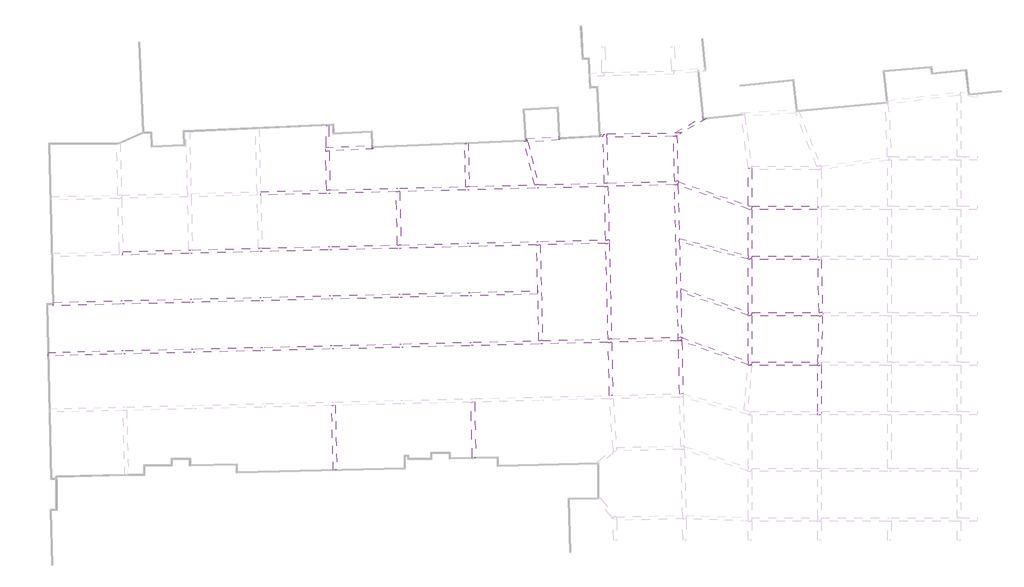
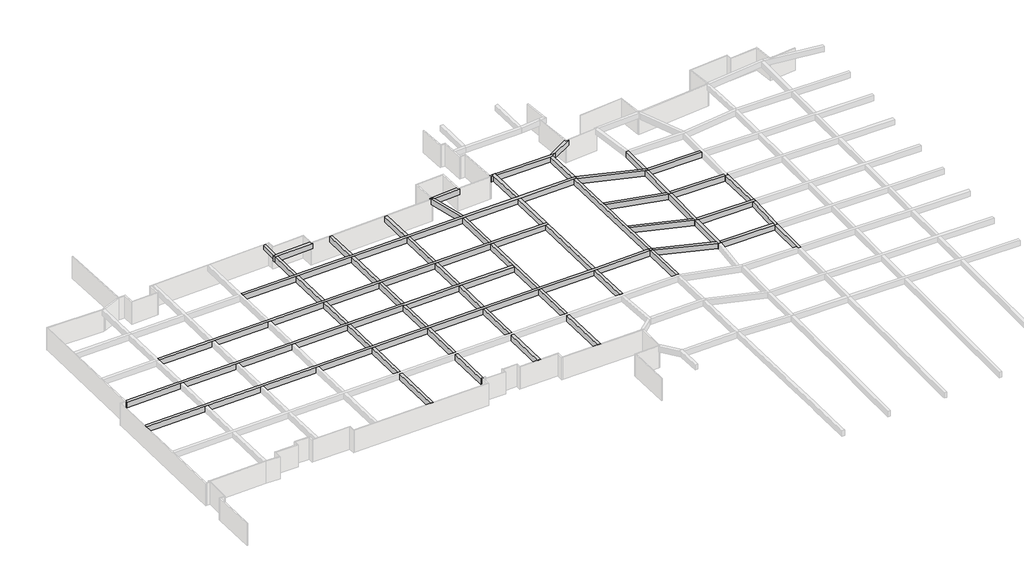
# One storey, part 17 of 20: 39 beams.
"""IFC4 building model written with IfcOpenShell, lengths in millimetres."""

from ifc_helpers import new_model, si_unit, frame, origin, place, context, project, spatial, polyline, outline, extrude, faceted_brep, element, save

model = new_model("IFC4")

# Units and contexts
model_context = context("Model", 3, world=origin())
ifc_project = project(units=[si_unit("LENGTHUNIT", "METRE", prefix="MILLI")], contexts=[model_context])

# Site, building, storey
site = spatial("IfcSite", under=ifc_project)
building = spatial("IfcBuilding", under=site)
storey = spatial("IfcBuildingStorey", under=building, Name="户型图", Elevation=0.0)

# Beams
placement = place(None, origin())
element("IfcBeam", 1, ObjectType="混凝土 - 矩形梁 : KL_beam", at=placement, inside=storey, context=model_context, shape_type="Brep", body=[
    faceted_brep([(46399.9946479, 182003.2647661, 3300.0), (46391.4589732, 182342.894025, 3300.0), (46389.9448891, 182403.1384991, 3300.0), (45990.0711561, 182393.0887404, 3300.0), (38313.3533834, 182200.154934, 3300.0), (37913.4796504, 182190.1051752, 3300.0), (30327.3489539, 181999.4480332, 3300.0), (29917.7537876, 181989.1539522, 3300.0), (22388.2477985, 181799.9199209, 3300.0), (21988.3737022, 181789.8701531, 3300.0), (14385.2020605, 181598.7847323, 3300.0), (13985.327054, 181588.7349416, 3300.0), (6399.8057805, 181398.0931157, 3300.0), (5999.9320475, 181388.043357, 3300.0), (-1606.785957, 181196.8688079, 3300.0), (-1597.0758138, 180796.9865396, 3300.0), (6009.5809432, 180988.1595494, 3300.0), (6409.4554783, 180998.2093283, 3300.0), (13994.367621, 181188.8358453, 3300.0), (14394.2426275, 181198.885636, 3300.0), (21997.9864051, 181389.9854358, 3300.0), (22397.8602787, 181400.0351981, 3300.0), (29976.8508171, 181590.5128914, 3300.0), (30376.7246906, 181600.5626536, 3300.0), (37923.3235545, 181790.2262686, 3300.0), (38323.1974993, 181800.2760327, 3300.0), (45975.016058, 181992.5840638, 3300.0), (46374.889791, 182002.6338225, 3300.0), (46399.9946479, 182003.2647661, 2500.0), (-1597.0758138, 180796.9865396, 2500.0), (6009.5809432, 180988.1595494, 2500.0), (6409.4554783, 180998.2093283, 2500.0), (13994.367621, 181188.8358453, 2500.0), (14394.2426275, 181198.885636, 2500.0), (21997.9864051, 181389.9854358, 2500.0), (22397.8602787, 181400.0351981, 2500.0), (29976.8508171, 181590.5128914, 2500.0), (30376.7246906, 181600.5626536, 2500.0), (37923.3235545, 181790.2262686, 2500.0), (38323.1974993, 181800.2760327, 2500.0), (45975.016058, 181992.5840638, 2500.0), (46374.889791, 182002.6338225, 2500.0), (46389.9448891, 182403.1384991, 2500.0), (46391.4589732, 182342.894025, 2500.0), (-1606.785957, 181196.8688079, 2500.0), (5999.9320475, 181388.043357, 2500.0), (6399.8057805, 181398.0931157, 2500.0), (13985.327054, 181588.7349416, 2500.0), (14385.2020605, 181598.7847323, 2500.0), (21988.3737022, 181789.8701531, 2500.0), (22388.2477985, 181799.9199209, 2500.0), (29917.7537876, 181989.1539522, 2500.0), (30327.3489539, 181999.4480332, 2500.0), (37913.4796504, 182190.1051752, 2500.0), (38313.3533834, 182200.154934, 2500.0), (45990.0711561, 182393.0887404, 2500.0)], [[[0, 1, 2, 3, 4, 5, 6, 7, 8, 9, 10, 11, 12, 13, 14, 15, 16, 17, 18, 19, 20, 21, 22, 23, 24, 25, 26, 27]], [[28, 0, 27, 26, 25, 24, 23, 22, 21, 20, 19, 18, 17, 16, 15, 29, 30, 31, 32, 33, 34, 35, 36, 37, 38, 39, 40, 41]], [[42, 43, 28, 41, 40, 39, 38, 37, 36, 35, 34, 33, 32, 31, 30, 29, 44, 45, 46, 47, 48, 49, 50, 51, 52, 53, 54, 55]], [[2, 42, 55, 54, 53, 52, 51, 50, 49, 48, 47, 46, 45, 44, 14, 13, 12, 11, 10, 9, 8, 7, 6, 5, 4, 3]], [[15, 14, 44, 29]], [[2, 1, 0, 28, 43, 42]]]),
])
element("IfcBeam", 2, ObjectType="混凝土 - 矩形梁 : KL_beam", at=placement, inside=storey, context=model_context, shape_type="Brep", body=[
    faceted_brep([(38480.8232268, 175260.5053635, 3300.0), (38471.1849707, 175660.3892266, 3300.0), (38071.3011075, 175650.7509705, 3300.0), (30525.6842312, 175468.8816956, 3300.0), (30125.8003608, 175459.2434392, 3300.0), (22546.6203468, 175276.5652041, 3300.0), (22146.7364764, 175266.9269478, 3300.0), (14532.4960637, 175083.4036646, 3300.0), (14132.6117538, 175073.7653977, 3300.0), (6550.7038885, 174891.0214142, 3300.0), (6150.8198357, 174881.3831535, 3300.0), (-1448.98219, 174698.2078735, 3300.0), (-1848.8660596, 174688.5696172, 3300.0), (-9443.7780087, 174505.5122009, 3300.0), (-9843.6618727, 174495.8739447, 3300.0), (-17442.3866011, 174312.7246305, 3300.0), (-17432.8215196, 173912.8390036, 3300.0), (-9834.048465, 174095.9894827, 3300.0), (-9434.164601, 174105.6277388, 3300.0), (-1839.1559197, 174288.6874866, 3300.0), (-1439.2720501, 174298.3257429, 3300.0), (6160.0686563, 174481.4899039, 3300.0), (6559.9527091, 174491.1281646, 3300.0), (14141.6523021, 174673.8671282, 3300.0), (14541.5366119, 174683.5053951, 3300.0), (22156.450981, 174867.0449224, 3300.0), (22556.3348514, 174876.6831788, 3300.0), (30135.5148654, 175059.3614139, 3300.0), (30535.3987358, 175068.9996702, 3300.0), (38080.9377827, 175250.8670692, 3300.0), (38480.8232268, 175260.5053635, 2500.0), (-17432.8215196, 173912.8390036, 2500.0), (-9834.048465, 174095.9894827, 2500.0), (-9434.164601, 174105.6277388, 2500.0), (-1839.1559197, 174288.6874866, 2500.0), (-1439.2720501, 174298.3257429, 2500.0), (6160.0686563, 174481.4899039, 2500.0), (6559.9527091, 174491.1281646, 2500.0), (14141.6523021, 174673.8671282, 2500.0), (14541.5366119, 174683.5053951, 2500.0), (22156.450981, 174867.0449224, 2500.0), (22556.3348514, 174876.6831788, 2500.0), (30135.5148654, 175059.3614139, 2500.0), (30535.3987358, 175068.9996702, 2500.0), (38080.9377827, 175250.8670692, 2500.0), (38471.1849707, 175660.3892266, 2500.0), (-17442.3866011, 174312.7246305, 2500.0), (-9843.6618727, 174495.8739447, 2500.0), (-9443.7780087, 174505.5122009, 2500.0), (-1848.8660596, 174688.5696172, 2500.0), (-1448.98219, 174698.2078735, 2500.0), (6150.8198357, 174881.3831535, 2500.0), (6550.7038885, 174891.0214142, 2500.0), (14132.6117538, 175073.7653977, 2500.0), (14532.4960637, 175083.4036646, 2500.0), (22146.7364764, 175266.9269478, 2500.0), (22546.6203468, 175276.5652041, 2500.0), (30125.8003608, 175459.2434392, 2500.0), (30525.6842312, 175468.8816956, 2500.0), (38071.3011075, 175650.7509705, 2500.0)], [[[0, 1, 2, 3, 4, 5, 6, 7, 8, 9, 10, 11, 12, 13, 14, 15, 16, 17, 18, 19, 20, 21, 22, 23, 24, 25, 26, 27, 28, 29]], [[30, 0, 29, 28, 27, 26, 25, 24, 23, 22, 21, 20, 19, 18, 17, 16, 31, 32, 33, 34, 35, 36, 37, 38, 39, 40, 41, 42, 43, 44]], [[45, 30, 44, 43, 42, 41, 40, 39, 38, 37, 36, 35, 34, 33, 32, 31, 46, 47, 48, 49, 50, 51, 52, 53, 54, 55, 56, 57, 58, 59]], [[1, 45, 59, 58, 57, 56, 55, 54, 53, 52, 51, 50, 49, 48, 47, 46, 15, 14, 13, 12, 11, 10, 9, 8, 7, 6, 5, 4, 3, 2]], [[16, 15, 46, 31]], [[1, 0, 30, 45]]]),
])
element("IfcBeam", 3, ObjectType="混凝土 - 矩形梁 : KL_beam", at=placement, inside=storey, context=model_context, shape_type="Brep", body=[
    faceted_brep([(-25454.7766609, 168469.9429507, 3300.0), (-25454.7766609, 168469.9429507, 2500.0), (-25445.2115795, 168070.0573306, 2500.0), (-25445.2115795, 168070.0573306, 3300.0), (-17696.541926, 168255.4019703, 3300.0), (-17296.6562991, 168264.9670519, 3300.0), (-9698.2373562, 168446.7177632, 3300.0), (-9298.3517331, 168456.2828447, 3300.0), (-1701.9427196, 168637.9854794, 3300.0), (-1302.0570732, 168647.5505615, 3300.0), (6290.7968198, 168829.1681594, 3300.0), (6690.682565, 168838.7332438, 3300.0), (14269.4696311, 169020.0143696, 3300.0), (14669.3555953, 169029.5794592, 3300.0), (22293.8325295, 169211.9534658, 3300.0), (22693.7181776, 169221.5185479, 3300.0), (30272.9318843, 169402.8098788, 3300.0), (30263.2173792, 169802.6919248, 3300.0), (22684.0036725, 169621.4005939, 3300.0), (22284.1180244, 169611.8355118, 3300.0), (14660.3150494, 169429.477626, 3300.0), (14260.4290852, 169419.9125364, 3300.0), (6681.4337459, 169238.6264288, 3300.0), (6281.5480006, 169229.0613444, 3300.0), (-1311.7672135, 169047.4327119, 3300.0), (-1711.65286, 169037.8676298, 3300.0), (-9307.9651408, 168856.1673089, 3300.0), (-9707.8507639, 168846.6022274, 3300.0), (-17306.2945554, 168664.8509217, 3300.0), (-17706.1801823, 168655.2858401, 3300.0), (-17696.541926, 168255.4019703, 2500.0), (-17296.6562991, 168264.9670519, 2500.0), (-9698.2373562, 168446.7177632, 2500.0), (-9298.3517331, 168456.2828447, 2500.0), (-1701.9427196, 168637.9854794, 2500.0), (-1302.0570732, 168647.5505615, 2500.0), (6290.7968198, 168829.1681594, 2500.0), (6690.682565, 168838.7332438, 2500.0), (14269.4696311, 169020.0143696, 2500.0), (14669.3555953, 169029.5794592, 2500.0), (22293.8325295, 169211.9534658, 2500.0), (22693.7181776, 169221.5185479, 2500.0), (30272.9318843, 169402.8098788, 2500.0), (-17706.1801823, 168655.2858401, 2500.0), (-17306.2945554, 168664.8509217, 2500.0), (-9707.8507639, 168846.6022274, 2500.0), (-9307.9651408, 168856.1673089, 2500.0), (-1711.65286, 169037.8676298, 2500.0), (-1311.7672135, 169047.4327119, 2500.0), (6281.5480006, 169229.0613444, 2500.0), (6681.4337459, 169238.6264288, 2500.0), (14260.4290852, 169419.9125364, 2500.0), (14660.3150494, 169429.477626, 2500.0), (22284.1180244, 169611.8355118, 2500.0), (22684.0036725, 169621.4005939, 2500.0), (30263.2173792, 169802.6919248, 2500.0)], [[[0, 1, 2, 3]], [[0, 3, 4, 5, 6, 7, 8, 9, 10, 11, 12, 13, 14, 15, 16, 17, 18, 19, 20, 21, 22, 23, 24, 25, 26, 27, 28, 29]], [[3, 2, 30, 31, 32, 33, 34, 35, 36, 37, 38, 39, 40, 41, 42, 16, 15, 14, 13, 12, 11, 10, 9, 8, 7, 6, 5, 4]], [[2, 1, 43, 44, 45, 46, 47, 48, 49, 50, 51, 52, 53, 54, 55, 42, 41, 40, 39, 38, 37, 36, 35, 34, 33, 32, 31, 30]], [[1, 0, 29, 28, 27, 26, 25, 24, 23, 22, 21, 20, 19, 18, 17, 55, 54, 53, 52, 51, 50, 49, 48, 47, 46, 45, 44, 43]], [[17, 16, 42, 55]]]),
])
element("IfcBeam", 4, ObjectType="混凝土 - 矩形梁 : KL_beam", at=placement, inside=storey, context=model_context, shape_type="Brep", body=[
    faceted_brep([(-26015.3324902, 162703.953657, 3300.0), (-26015.3324902, 162703.953657, 2500.0), (-26005.697396, 162304.0697176, 2500.0), (-26005.697396, 162304.0697176, 3300.0), (-17558.0050844, 162507.6145551, 3300.0), (-17158.121145, 162517.2496493, 3300.0), (-9560.0913428, 162700.3221009, 3300.0), (-9160.2074028, 162709.9571951, 3300.0), (-1562.4406466, 162893.0233086, 3300.0), (-1162.5567002, 162902.658403, 3300.0), (6423.6389192, 163085.4457131, 3300.0), (6823.5230451, 163095.0808118, 3300.0), (14399.2887031, 163277.6168149, 3300.0), (14799.1730844, 163287.2519198, 3300.0), (22433.2952474, 163471.1940069, 3300.0), (22833.1791946, 163480.8291013, 3300.0), (30412.3606645, 163663.4474074, 3300.0), (30812.2446118, 163673.0825018, 3300.0), (38355.4870343, 163854.8348664, 3300.0), (38755.3709798, 163864.4699608, 3300.0), (46425.7655975, 164049.2860227, 3300.0), (46825.6495368, 164058.9211169, 3300.0), (46817.5217221, 164396.248649, 3300.0), (46816.0144426, 164458.8050563, 3300.0), (46653.1511282, 164454.8809093, 3300.0), (46378.5988907, 164448.2656481, 3300.0), (38745.7708888, 164264.3547435, 3300.0), (38345.8869495, 164254.7196493, 3300.0), (30802.5301072, 164072.9645278, 3300.0), (30402.6461599, 164063.3294334, 3300.0), (22823.46469, 163880.7111273, 3300.0), (22423.5807428, 163871.0760328, 3300.0), (14790.1325363, 163687.1501845, 3300.0), (14390.2481549, 163677.5150797, 3300.0), (6814.2742245, 163494.9740584, 3300.0), (6414.3900986, 163485.3389596, 3300.0), (-1172.2668401, 163302.5405341, 3300.0), (-1572.1507865, 163292.9054397, 3300.0), (-9169.8208105, 163109.841657, 3300.0), (-9569.7047505, 163100.2065627, 3300.0), (-17167.7594012, 162917.1335125, 3300.0), (-17567.6433405, 162907.4984183, 3300.0), (-17558.0050844, 162507.6145551, 2500.0), (-17158.121145, 162517.2496493, 2500.0), (-9560.0913428, 162700.3221009, 2500.0), (-9160.2074028, 162709.9571951, 2500.0), (-1562.4406466, 162893.0233086, 2500.0), (-1162.5567002, 162902.658403, 2500.0), (6423.6389192, 163085.4457131, 2500.0), (6823.5230451, 163095.0808118, 2500.0), (14399.2887031, 163277.6168149, 2500.0), (14799.1730844, 163287.2519198, 2500.0), (22433.2952474, 163471.1940069, 2500.0), (22833.1791946, 163480.8291013, 2500.0), (30412.3606645, 163663.4474074, 2500.0), (30812.2446118, 163673.0825018, 2500.0), (38355.4870343, 163854.8348664, 2500.0), (38755.3709798, 163864.4699608, 2500.0), (46425.7655975, 164049.2860227, 2500.0), (46825.6495368, 164058.9211169, 2500.0), (-17567.6433405, 162907.4984183, 2500.0), (-17167.7594012, 162917.1335125, 2500.0), (-9569.7047505, 163100.2065627, 2500.0), (-9169.8208105, 163109.841657, 2500.0), (-1572.1507865, 163292.9054397, 2500.0), (-1172.2668401, 163302.5405341, 2500.0), (6414.3900986, 163485.3389596, 2500.0), (6814.2742245, 163494.9740584, 2500.0), (14390.2481549, 163677.5150797, 2500.0), (14790.1325363, 163687.1501845, 2500.0), (22423.5807428, 163871.0760328, 2500.0), (22823.46469, 163880.7111273, 2500.0), (30402.6461599, 164063.3294334, 2500.0), (30802.5301072, 164072.9645278, 2500.0), (38345.8869495, 164254.7196493, 2500.0), (38745.7708888, 164264.3547435, 2500.0), (46378.5988907, 164448.2656481, 2500.0), (46653.1511282, 164454.8809093, 2500.0), (46816.0144426, 164458.8050563, 2500.0), (46817.5217221, 164396.248649, 2500.0)], [[[0, 1, 2, 3]], [[0, 3, 4, 5, 6, 7, 8, 9, 10, 11, 12, 13, 14, 15, 16, 17, 18, 19, 20, 21, 22, 23, 24, 25, 26, 27, 28, 29, 30, 31, 32, 33, 34, 35, 36, 37, 38, 39, 40, 41]], [[3, 2, 42, 43, 44, 45, 46, 47, 48, 49, 50, 51, 52, 53, 54, 55, 56, 57, 58, 59, 21, 20, 19, 18, 17, 16, 15, 14, 13, 12, 11, 10, 9, 8, 7, 6, 5, 4]], [[2, 1, 60, 61, 62, 63, 64, 65, 66, 67, 68, 69, 70, 71, 72, 73, 74, 75, 76, 77, 78, 79, 59, 58, 57, 56, 55, 54, 53, 52, 51, 50, 49, 48, 47, 46, 45, 44, 43, 42]], [[1, 0, 41, 40, 39, 38, 37, 36, 35, 34, 33, 32, 31, 30, 29, 28, 27, 26, 25, 24, 23, 78, 77, 76, 75, 74, 73, 72, 71, 70, 69, 68, 67, 66, 65, 64, 63, 62, 61, 60]], [[23, 22, 21, 59, 79, 78]]]),
])
element("IfcBeam", 5, ObjectType="混凝土 - 矩形梁 : KL_beam", at=placement, inside=storey, context=model_context, shape_type="Brep", body=[
    faceted_brep([(11202.8971175, 186239.6731287, 3300.0), (11197.5533917, 186359.5540888, 3300.0), (11190.8059936, 186510.9249863, 3300.0), (6232.0, 186289.8848868, 3300.0), (5932.0, 186276.5123068, 3300.0), (5877.1348957, 186274.0666802, 3300.0), (5887.1865495, 185874.1175417, 3300.0), (6286.8651043, 185891.9333198, 3300.0), (11328.4993729, 186116.6655117, 3300.0), (11322.7780776, 186245.0168545, 3300.0), (11328.4993729, 186116.6655117, 2500.0), (5887.1865495, 185874.1175417, 2500.0), (6286.8651043, 185891.9333198, 2500.0), (11190.8059936, 186510.9249863, 2500.0), (11202.8971175, 186239.6731287, 2500.0), (11322.7780776, 186245.0168545, 2500.0), (5877.1348957, 186274.0666802, 2500.0)], [[[0, 1, 2, 3, 4, 5, 6, 7, 8, 9]], [[10, 8, 7, 6, 11, 12]], [[13, 14, 15, 10, 12, 11, 16]], [[2, 13, 16, 5, 4, 3]], [[8, 10, 15, 9]], [[0, 14, 13, 2, 1]], [[14, 0, 9, 15]], [[6, 5, 16, 11]]]),
])
element("IfcBeam", 6, ObjectType="混凝土 - 矩形梁 : KL_beam", at=placement, inside=storey, context=model_context, shape_type="SweptSolid", body=[
    extrude(outline(polyline([(5887.1865495, 185874.1175417), (6286.8651043, 185891.9333198), (6399.8057805, 181398.0931157), (5999.9320475, 181388.043357), (5887.1865495, 185874.1175417)])), frame((0.0, 0.0, 2500.0), z_axis=(0.0, 0.0, 1.0), x_axis=(1.0, 0.0, 0.0)), (0.0, 0.0, 1.0), 800.0),
])
element("IfcBeam", 7, ObjectType="混凝土 - 矩形梁 : KL_beam", at=placement, inside=storey, context=model_context, shape_type="SweptSolid", body=[
    extrude(outline(polyline([(7144.9385656, 149197.9687644), (6745.0455057, 149188.7199481), (6573.7901577, 156593.3242925), (6973.6759029, 156602.8893769), (7144.9385656, 149197.9687644)])), frame((0.0, 0.0, 2500.0), z_axis=(0.0, 0.0, 1.0), x_axis=(1.0, 0.0, 0.0)), (0.0, 0.0, 1.0), 800.0),
    extrude(outline(polyline([(6009.5809432, 180988.1595494), (6409.4554783, 180998.2093283), (6550.7038885, 174891.0214142), (6150.8198357, 174881.3831535), (6009.5809432, 180988.1595494)])), frame((0.0, 0.0, 2500.0), z_axis=(0.0, 0.0, 1.0), x_axis=(1.0, 0.0, 0.0)), (0.0, 0.0, 1.0), 800.0),
    extrude(outline(polyline([(6160.0686563, 174481.4899039), (6559.9527091, 174491.1281646), (6681.4337459, 169238.6264288), (6281.5480006, 169229.0613444), (6160.0686563, 174481.4899039)])), frame((0.0, 0.0, 2500.0), z_axis=(0.0, 0.0, 1.0), x_axis=(1.0, 0.0, 0.0)), (0.0, 0.0, 1.0), 800.0),
    extrude(outline(polyline([(6290.7968198, 168829.1681594), (6690.682565, 168838.7332438), (6814.2742245, 163494.9740584), (6414.3900986, 163485.3389596), (6290.7968198, 168829.1681594)])), frame((0.0, 0.0, 2500.0), z_axis=(0.0, 0.0, 1.0), x_axis=(1.0, 0.0, 0.0)), (0.0, 0.0, 1.0), 800.0),
    extrude(outline(polyline([(6423.6389192, 163085.4457131), (6823.5230451, 163095.0808118), (6964.4270838, 157002.7825619), (6564.5413385, 156993.2174775), (6423.6389192, 163085.4457131)])), frame((0.0, 0.0, 2500.0), z_axis=(0.0, 0.0, 1.0), x_axis=(1.0, 0.0, 0.0)), (0.0, 0.0, 1.0), 800.0),
])
element("IfcBeam", 8, ObjectType="混凝土 - 矩形梁 : KL_beam", at=placement, inside=storey, context=model_context, shape_type="SweptSolid", body=[
    extrude(outline(polyline([(15083.9383621, 150690.9869029), (14684.0405394, 150681.9463647), (14546.0902706, 156784.0180707), (14945.9762348, 156793.5831603), (15083.9383621, 150690.9869029)])), frame((0.0, 0.0, 2500.0), z_axis=(0.0, 0.0, 1.0), x_axis=(1.0, 0.0, 0.0)), (0.0, 0.0, 1.0), 800.0),
    extrude(outline(polyline([(13877.4875012, 186358.8937082), (14277.1869201, 186376.7104164), (14385.2020605, 181598.7847323), (13985.327054, 181588.7349416), (13877.4875012, 186358.8937082)])), frame((0.0, 0.0, 2500.0), z_axis=(0.0, 0.0, 1.0), x_axis=(1.0, 0.0, 0.0)), (0.0, 0.0, 1.0), 800.0),
    extrude(outline(polyline([(13994.367621, 181188.8358453), (14394.2426275, 181198.885636), (14532.4960637, 175083.4036646), (14132.6117538, 175073.7653977), (13994.367621, 181188.8358453)])), frame((0.0, 0.0, 2500.0), z_axis=(0.0, 0.0, 1.0), x_axis=(1.0, 0.0, 0.0)), (0.0, 0.0, 1.0), 800.0),
    extrude(outline(polyline([(14141.6523021, 174673.8671282), (14541.5366119, 174683.5053951), (14660.3150494, 169429.477626), (14260.4290852, 169419.9125364), (14141.6523021, 174673.8671282)])), frame((0.0, 0.0, 2500.0), z_axis=(0.0, 0.0, 1.0), x_axis=(1.0, 0.0, 0.0)), (0.0, 0.0, 1.0), 800.0),
    extrude(outline(polyline([(14269.4696311, 169020.0143696), (14669.3555953, 169029.5794592), (14790.1325363, 163687.1501845), (14390.2481549, 163677.5150797), (14269.4696311, 169020.0143696)])), frame((0.0, 0.0, 2500.0), z_axis=(0.0, 0.0, 1.0), x_axis=(1.0, 0.0, 0.0)), (0.0, 0.0, 1.0), 800.0),
    extrude(outline(polyline([(14399.2887031, 163277.6168149), (14799.1730844, 163287.2519198), (14936.9356889, 157193.4813271), (14537.0497247, 157183.9162375), (14399.2887031, 163277.6168149)])), frame((0.0, 0.0, 2500.0), z_axis=(0.0, 0.0, 1.0), x_axis=(1.0, 0.0, 0.0)), (0.0, 0.0, 1.0), 800.0),
])
element("IfcBeam", 9, ObjectType="混凝土 - 矩形梁 : KL_beam", at=placement, inside=storey, context=model_context, shape_type="SweptSolid", body=[
    extrude(outline(polyline([(23146.5170418, 150582.7783735), (22746.6350237, 150573.0638691), (22591.0748231, 156976.4504274), (22990.9604712, 156986.0155095), (23146.5170418, 150582.7783735)])), frame((0.0, 0.0, 2500.0), z_axis=(0.0, 0.0, 1.0), x_axis=(1.0, 0.0, 0.0)), (0.0, 0.0, 1.0), 800.0),
    extrude(outline(polyline([(21997.9864051, 181389.9854358), (22397.8602787, 181400.0351981), (22546.6203468, 175276.5652041), (22146.7364764, 175266.9269478), (21997.9864051, 181389.9854358)])), frame((0.0, 0.0, 2500.0), z_axis=(0.0, 0.0, 1.0), x_axis=(1.0, 0.0, 0.0)), (0.0, 0.0, 1.0), 800.0),
    extrude(outline(polyline([(22156.450981, 174867.0449224), (22556.3348514, 174876.6831788), (22684.0036725, 169621.4005939), (22284.1180244, 169611.8355118), (22156.450981, 174867.0449224)])), frame((0.0, 0.0, 2500.0), z_axis=(0.0, 0.0, 1.0), x_axis=(1.0, 0.0, 0.0)), (0.0, 0.0, 1.0), 800.0),
    extrude(outline(polyline([(22293.8325295, 169211.9534658), (22693.7181776, 169221.5185479), (22823.46469, 163880.7111273), (22423.5807428, 163871.0760328), (22293.8325295, 169211.9534658)])), frame((0.0, 0.0, 2500.0), z_axis=(0.0, 0.0, 1.0), x_axis=(1.0, 0.0, 0.0)), (0.0, 0.0, 1.0), 800.0),
    extrude(outline(polyline([(22433.2952474, 163471.1940069), (22833.1791946, 163480.8291013), (22981.2459661, 157385.8975556), (22581.360318, 157376.3324735), (22433.2952474, 163471.1940069)])), frame((0.0, 0.0, 2500.0), z_axis=(0.0, 0.0, 1.0), x_axis=(1.0, 0.0, 0.0)), (0.0, 0.0, 1.0), 800.0),
])
element("IfcBeam", 10, ObjectType="混凝土 - 矩形梁 : KL_beam", at=placement, inside=storey, context=model_context, shape_type="SweptSolid", body=[
    extrude(outline(polyline([(31149.865998, 149775.4387741), (30749.9839799, 149765.7242696), (30570.1741778, 157167.3068404), (30970.0598259, 157176.8719225), (31149.865998, 149775.4387741)])), frame((0.0, 0.0, 2500.0), z_axis=(0.0, 0.0, 1.0), x_axis=(1.0, 0.0, 0.0)), (0.0, 0.0, 1.0), 800.0),
    extrude(outline(polyline([(29976.8508171, 181590.5128914), (30376.7246906, 181600.5626536), (30525.6842312, 175468.8816956), (30125.8003608, 175459.2434392), (29976.8508171, 181590.5128914)])), frame((0.0, 0.0, 2500.0), z_axis=(0.0, 0.0, 1.0), x_axis=(1.0, 0.0, 0.0)), (0.0, 0.0, 1.0), 800.0),
    extrude(outline(polyline([(30135.5148654, 175059.3614139), (30535.3987358, 175068.9996702), (30802.5301072, 164072.9645278), (30402.6461599, 164063.3294334), (30135.5148654, 175059.3614139)])), frame((0.0, 0.0, 2500.0), z_axis=(0.0, 0.0, 1.0), x_axis=(1.0, 0.0, 0.0)), (0.0, 0.0, 1.0), 800.0),
    extrude(outline(polyline([(30412.3606645, 163663.4474074), (30812.2446118, 163673.0825018), (30960.3453208, 157576.7539685), (30560.4596727, 157567.1888864), (30412.3606645, 163663.4474074)])), frame((0.0, 0.0, 2500.0), z_axis=(0.0, 0.0, 1.0), x_axis=(1.0, 0.0, 0.0)), (0.0, 0.0, 1.0), 800.0),
])
element("IfcBeam", 11, ObjectType="混凝土 - 矩形梁 : KL_beam", at=placement, inside=storey, context=model_context, shape_type="SweptSolid", body=[
    extrude(outline(polyline([(21871.2322555, 186715.2170123), (22270.9216383, 186733.0332731), (22388.2477985, 181799.9199209), (21988.3737022, 181789.8701531), (21871.2322555, 186715.2170123)])), frame((0.0, 0.0, 2500.0), z_axis=(0.0, 0.0, 1.0), x_axis=(1.0, 0.0, 0.0)), (0.0, 0.0, 1.0), 800.0),
])
element("IfcBeam", 12, ObjectType="混凝土 - 矩形梁 : KL_beam", at=placement, inside=storey, context=model_context, shape_type="Brep", body=[
    faceted_brep([(29046.8770272, 187155.1924495, 3300.0), (28914.6125725, 187149.2967262, 3300.0), (28920.893079, 187029.4575233, 3300.0), (28668.7440041, 187018.2179111, 3300.0), (29917.7537876, 181989.1539522, 3300.0), (30327.3489539, 181999.4480332, 3300.0), (29109.3115678, 186903.8034674, 3300.0), (29917.7537876, 181989.1539522, 2500.0), (28668.7440041, 187018.2179111, 2500.0), (28914.6125725, 187149.2967262, 2500.0), (29046.8770272, 187155.1924495, 2500.0), (29109.3115678, 186903.8034674, 2500.0), (30327.3489539, 181999.4480332, 2500.0), (28920.893079, 187029.4575233, 2500.0)], [[[0, 1, 2, 3, 4, 5, 6]], [[7, 4, 3, 8]], [[9, 10, 11, 12, 7, 8, 13]], [[10, 0, 6, 5, 12, 11]], [[0, 10, 9, 1]], [[13, 2, 1, 9]], [[2, 13, 8, 3]], [[5, 4, 7, 12]]]),
])
element("IfcBeam", 13, ObjectType="混凝土 - 矩形梁 : KL_beam", at=placement, inside=storey, context=model_context, shape_type="Brep", body=[
    faceted_brep([(38171.3567272, 187850.1147578, 3300.0), (37771.4829941, 187840.0649991, 3300.0), (37779.036637, 187539.5101843, 3300.0), (37913.4796504, 182190.1051752, 3300.0), (38313.3533834, 182200.154934, 3300.0), (38180.8867031, 187470.9228612, 3300.0), (38171.3567272, 187850.1147578, 2500.0), (38313.3533834, 182200.154934, 2500.0), (38180.8867031, 187470.9228612, 2500.0), (37771.4829941, 187840.0649991, 2500.0), (37913.4796504, 182190.1051752, 2500.0), (37779.036637, 187539.5101843, 2500.0)], [[[0, 1, 2, 3, 4, 5]], [[6, 0, 5, 4, 7, 8]], [[9, 6, 8, 7, 10, 11]], [[1, 9, 11, 10, 3, 2]], [[4, 3, 10, 7]], [[1, 0, 6, 9]]]),
])
element("IfcBeam", 14, ObjectType="混凝土 - 矩形梁 : KL_beam", at=placement, inside=storey, context=model_context, shape_type="SweptSolid", body=[
    extrude(outline(polyline([(37421.6044199, 187787.8333432), (37771.4829941, 187840.0649991), (37779.036637, 187539.5101843), (37435.5618645, 187521.5094342), (37421.6044199, 187787.8333432)])), frame((0.0, 0.0, 2500.0), z_axis=(0.0, 0.0, 1.0), x_axis=(1.0, 0.0, 0.0)), (0.0, 0.0, 1.0), 800.0),
])
element("IfcBeam", 15, ObjectType="混凝土 - 矩形梁 : KL_beam", at=placement, inside=storey, context=model_context, shape_type="Brep", body=[
    faceted_brep([(32673.3455379, 187271.9322521, 3300.0), (32667.0652231, 187391.7677963, 3300.0), (32658.6168776, 187552.9718316, 3300.0), (28907.2046904, 187290.6475371, 3300.0), (28914.6125725, 187149.2967262, 3300.0), (29046.8770272, 187155.1924495, 3300.0), (29109.3115678, 186903.8034674, 3300.0), (32799.2803699, 187161.8312219, 3300.0), (32793.1810821, 187278.2125669, 3300.0), (32799.2803699, 187161.8312219, 2500.0), (29109.3115678, 186903.8034674, 2500.0), (32658.6168776, 187552.9718316, 2500.0), (32673.3455379, 187271.9322521, 2500.0), (32793.1810821, 187278.2125669, 2500.0), (29046.8770272, 187155.1924495, 2500.0), (28914.6125725, 187149.2967262, 2500.0), (28907.2046904, 187290.6475371, 2500.0)], [[[0, 1, 2, 3, 4, 5, 6, 7, 8]], [[9, 7, 6, 10]], [[11, 12, 13, 9, 10, 14, 15, 16]], [[2, 11, 16, 3]], [[7, 9, 13, 8]], [[0, 12, 11, 2, 1]], [[3, 16, 15, 4]], [[5, 14, 10, 6]], [[14, 5, 4, 15]], [[12, 0, 8, 13]]]),
    faceted_brep([(28606.3094635, 187269.6068931, 3300.0), (28606.3094635, 187269.6068931, 2500.0), (28639.2380636, 187137.021834, 2500.0), (28639.2380636, 187137.021834, 3300.0), (28787.4787695, 187282.2754851, 2500.0), (28787.4787695, 187282.2754851, 3300.0), (28794.7279523, 187143.9528373, 3300.0), (28794.7279523, 187143.9528373, 2500.0)], [[[0, 1, 2, 3]], [[4, 5, 6, 7]], [[1, 0, 5, 4]], [[5, 0, 3, 6]], [[1, 4, 7, 2]], [[6, 3, 2, 7]]]),
])
element("IfcBeam", 16, ObjectType="混凝土 - 矩形梁 : KL_beam", at=placement, inside=storey, context=model_context, shape_type="Brep", body=[
    faceted_brep([(38283.9984147, 187872.2517247, 3300.0), (38284.4833137, 187852.9578926, 3300.0), (38171.3567272, 187850.1147578, 3300.0), (38178.6366189, 187560.452332, 3300.0), (38180.8867031, 187470.9228612, 3300.0), (45860.0253576, 187567.5312694, 3300.0), (46109.0857553, 187570.6646063, 3300.0), (46257.9441503, 187655.3669007, 3300.0), (46828.0086678, 187979.7407633, 3300.0), (46000.9142447, 187969.3353937, 3300.0), (38180.8867031, 187470.9228612, 2500.0), (45860.0253576, 187567.5312694, 2500.0), (46109.0857553, 187570.6646063, 2500.0), (38284.4833137, 187852.9578926, 2500.0), (38283.9984147, 187872.2517247, 2500.0), (46000.9142447, 187969.3353937, 2500.0), (46828.0086678, 187979.7407633, 2500.0), (46257.9441503, 187655.3669007, 2500.0), (38178.6366189, 187560.452332, 2500.0), (38171.3567272, 187850.1147578, 2500.0)], [[[0, 1, 2, 3, 4, 5, 6, 7, 8, 9]], [[4, 10, 11, 12, 6, 5]], [[13, 14, 15, 16, 17, 12, 11, 10, 18, 19]], [[14, 0, 9, 8, 16, 15]], [[1, 13, 19, 2]], [[13, 1, 0, 14]], [[10, 4, 3, 2, 19, 18]], [[8, 7, 6, 12, 17, 16]]]),
])
element("IfcBeam", 17, ObjectType="混凝土 - 矩形梁 : KL_beam", at=placement, inside=storey, context=model_context, shape_type="SweptSolid", body=[
    extrude(outline(polyline([(49187.5690842, 189782.5819775), (49211.8887729, 189530.9836906), (49631.7675174, 189575.1147249), (46828.0086678, 187979.7407633), (46000.9142447, 187969.3353937), (49187.5690842, 189782.5819775)])), frame((0.0, 0.0, 2500.0), z_axis=(0.0, 0.0, 1.0), x_axis=(1.0, 0.0, 0.0)), (0.0, 0.0, 1.0), 800.0),
])
element("IfcBeam", 18, ObjectType="混凝土 - 矩形梁 : KL_beam", at=placement, inside=storey, context=model_context, shape_type="SweptSolid", body=[
    extrude(outline(polyline([(46389.9448891, 182403.1384991), (45990.0711561, 182393.0887404), (45860.0253576, 187567.5312694), (46109.0857553, 187570.6646063), (46257.9441503, 187655.3669007), (46389.9448891, 182403.1384991)])), frame((0.0, 0.0, 2500.0), z_axis=(0.0, 0.0, 1.0), x_axis=(1.0, 0.0, 0.0)), (0.0, 0.0, 1.0), 800.0),
])
element("IfcBeam", 19, ObjectType="混凝土 - 矩形梁 : KL_beam", at=placement, inside=storey, context=model_context, shape_type="SweptSolid", body=[
    extrude(outline(polyline([(38471.1849707, 175660.3892266), (38071.3011075, 175650.7509705), (37923.3235545, 181790.2262686), (38323.1974993, 181800.2760327), (38471.1849707, 175660.3892266)])), frame((0.0, 0.0, 2500.0), z_axis=(0.0, 0.0, 1.0), x_axis=(1.0, 0.0, 0.0)), (0.0, 0.0, 1.0), 800.0),
])
element("IfcBeam", 20, ObjectType="混凝土 - 矩形梁 : KL_beam", at=placement, inside=storey, context=model_context, shape_type="SweptSolid", body=[
    extrude(outline(polyline([(38080.9377827, 175250.8670692), (38480.8216459, 175260.5053254), (38745.7708888, 164264.3547435), (38345.8869495, 164254.7196493), (38080.9377827, 175250.8670692)])), frame((0.0, 0.0, 2500.0), z_axis=(0.0, 0.0, 1.0), x_axis=(1.0, 0.0, 0.0)), (0.0, 0.0, 1.0), 800.0),
])
element("IfcBeam", 21, ObjectType="混凝土 - 矩形梁 : KL_beam", at=placement, inside=storey, context=model_context, shape_type="SweptSolid", body=[
    extrude(outline(polyline([(38355.4870343, 163854.8348664), (38755.3709798, 163864.4699608), (38901.2269429, 157766.6962307), (38501.3413227, 157757.1311493), (38355.4870343, 163854.8348664)])), frame((0.0, 0.0, 2500.0), z_axis=(0.0, 0.0, 1.0), x_axis=(1.0, 0.0, 0.0)), (0.0, 0.0, 1.0), 800.0),
])
element("IfcBeam", 22, ObjectType="混凝土 - 矩形梁 : KL_beam", at=placement, inside=storey, context=model_context, shape_type="Brep", body=[
    faceted_brep([(46825.6495368, 164058.9211169, 3300.0), (46425.7655975, 164049.2860227, 3300.0), (46572.7215317, 157950.1948781, 3300.0), (46972.607158, 157959.7599597, 3300.0), (46827.843133, 163967.8806096, 3300.0), (46825.6495368, 164058.9211169, 2500.0), (46972.607158, 157959.7599597, 2500.0), (46827.843133, 163967.8806096, 2500.0), (46425.7655975, 164049.2860227, 2500.0), (46572.7215317, 157950.1948781, 2500.0)], [[[0, 1, 2, 3, 4]], [[5, 0, 4, 3, 6, 7]], [[8, 5, 7, 6, 9]], [[1, 8, 9, 2]], [[1, 0, 5, 8]], [[3, 2, 9, 6]]]),
])
element("IfcBeam", 23, ObjectType="混凝土 - 矩形梁 : KL_beam", at=placement, inside=storey, context=model_context, shape_type="Brep", body=[
    faceted_brep([(46588.6289118, 164053.2101698, 3300.0), (46828.1478972, 163967.7718979, 3300.0), (46686.0772854, 169620.6743645, 3300.0), (46675.352285, 170047.4155508, 3300.0), (46540.6846864, 175405.7566657, 3300.0), (46530.2586661, 175820.6016162, 3300.0), (46376.8257377, 181925.6036927, 3300.0), (46374.889791, 182002.6338225, 3300.0), (46000.1209149, 181993.2150074, 3300.0), (45975.016058, 181992.5840638, 3300.0), (46425.9728249, 164049.2910158, 3300.0), (46828.1478972, 163967.7718979, 2500.0), (46686.0772854, 169620.6743645, 2500.0), (46675.352285, 170047.4155508, 2500.0), (46540.6846864, 175405.7566657, 2500.0), (46530.2586661, 175820.6016162, 2500.0), (46376.8257377, 181925.6036927, 2500.0), (46374.889791, 182002.6338225, 2500.0), (46588.6289118, 164053.2101698, 2500.0), (46425.9728249, 164049.2910158, 2500.0), (45975.016058, 181992.5840638, 2500.0), (46000.1209149, 181993.2150074, 2500.0)], [[[0, 1, 2, 3, 4, 5, 6, 7, 8, 9, 10]], [[1, 11, 12, 13, 14, 15, 16, 17, 7, 6, 5, 4, 3, 2]], [[11, 18, 19, 20, 21, 17, 16, 15, 14, 13, 12]], [[10, 9, 20, 19]], [[1, 0, 18, 11]], [[7, 17, 21, 20, 9, 8]], [[18, 0, 10, 19]]]),
])
element("IfcBeam", 24, ObjectType="混凝土 - 矩形梁 : KL_beam", at=placement, inside=storey, context=model_context, shape_type="Brep", body=[
    faceted_brep([(46391.4589732, 182342.894025, 3300.0), (46399.9946479, 182003.2647661, 3300.0), (46374.889791, 182002.6338225, 3300.0), (46376.8257377, 181925.6036927, 3300.0), (54450.0, 179196.4908844, 3300.0), (54850.0, 179061.2720612, 3300.0), (54850.0, 179140.0, 3300.0), (54850.0, 179483.5091156, 3300.0), (54450.0, 179618.7279388, 3300.0), (54850.0, 179061.2720612, 2500.0), (46376.8257377, 181925.6036927, 2500.0), (54450.0, 179196.4908844, 2500.0), (46399.9946479, 182003.2647661, 2500.0), (46391.4589732, 182342.894025, 2500.0), (54450.0, 179618.7279388, 2500.0), (54850.0, 179483.5091156, 2500.0), (54850.0, 179140.0, 2500.0), (46374.889791, 182002.6338225, 2500.0)], [[[0, 1, 2, 3, 4, 5, 6, 7, 8]], [[9, 5, 4, 3, 10, 11]], [[12, 13, 14, 15, 16, 9, 11, 10, 17]], [[13, 0, 8, 7, 15, 14]], [[12, 1, 0, 13]], [[1, 12, 17, 2]], [[3, 2, 17, 10]], [[7, 6, 5, 9, 16, 15]]]),
])
element("IfcBeam", 25, ObjectType="混凝土 - 矩形梁 : KL_beam", at=placement, inside=storey, context=model_context, shape_type="Brep", body=[
    faceted_brep([(54450.0, 173433.7428747, 3300.0), (54850.0, 173433.7428747, 3300.0), (54850.0, 173790.0, 3300.0), (54850.0, 179061.2720612, 3300.0), (54450.0, 179196.4908844, 3300.0), (54450.0, 173845.9883264, 3300.0), (54450.0, 173433.7428747, 2500.0), (54450.0, 179196.4908844, 2500.0), (54450.0, 173845.9883264, 2500.0), (54850.0, 173433.7428747, 2500.0), (54850.0, 179061.2720612, 2500.0), (54850.0, 173790.0, 2500.0)], [[[0, 1, 2, 3, 4, 5]], [[6, 0, 5, 4, 7, 8]], [[9, 6, 8, 7, 10, 11]], [[1, 9, 11, 10, 3, 2]], [[4, 3, 10, 7]], [[1, 0, 6, 9]]]),
])
element("IfcBeam", 26, ObjectType="混凝土 - 矩形梁 : KL_beam", at=placement, inside=storey, context=model_context, shape_type="SweptSolid", body=[
    extrude(outline(polyline([(54450.0, 173845.9883264), (54450.0, 173433.7428747), (46540.6846864, 175405.7566657), (46530.2586661, 175820.6016162), (54450.0, 173845.9883264)])), frame((0.0, 0.0, 2500.0), z_axis=(0.0, 0.0, 1.0), x_axis=(1.0, 0.0, 0.0)), (0.0, 0.0, 1.0), 800.0),
])
element("IfcBeam", 27, ObjectType="混凝土 - 矩形梁 : KL_beam", at=placement, inside=storey, context=model_context, shape_type="Brep", body=[
    faceted_brep([(54450.0, 166947.3413864, 3300.0), (54850.0, 166947.3413864, 3300.0), (54850.0, 167290.0, 3300.0), (54850.0, 173390.0, 3300.0), (54850.0, 173433.7428747, 3300.0), (54450.0, 173433.7428747, 3300.0), (54450.0, 167370.3896589, 3300.0), (54450.0, 166947.3413864, 2500.0), (54450.0, 173433.7428747, 2500.0), (54450.0, 167370.3896589, 2500.0), (54850.0, 166947.3413864, 2500.0), (54850.0, 173433.7428747, 2500.0), (54850.0, 173390.0, 2500.0), (54850.0, 167290.0, 2500.0)], [[[0, 1, 2, 3, 4, 5, 6]], [[7, 0, 6, 5, 8, 9]], [[10, 7, 9, 8, 11, 12, 13]], [[1, 10, 13, 12, 11, 4, 3, 2]], [[5, 4, 11, 8]], [[1, 0, 7, 10]]]),
])
element("IfcBeam", 28, ObjectType="混凝土 - 矩形梁 : KL_beam", at=placement, inside=storey, context=model_context, shape_type="SweptSolid", body=[
    extrude(outline(polyline([(54450.0, 167370.3896589), (54450.0, 166947.3413864), (46686.0772854, 169620.6743645), (46675.352285, 170047.4155508), (54450.0, 167370.3896589)])), frame((0.0, 0.0, 2500.0), z_axis=(0.0, 0.0, 1.0), x_axis=(1.0, 0.0, 0.0)), (0.0, 0.0, 1.0), 800.0),
])
element("IfcBeam", 29, ObjectType="混凝土 - 矩形梁 : KL_beam", at=placement, inside=storey, context=model_context, shape_type="Brep", body=[
    faceted_brep([(54450.0, 161248.9983884, 3300.0), (54850.0, 161248.9983884, 3300.0), (54850.0, 161590.0, 3300.0), (54850.0, 166890.0, 3300.0), (54850.0, 166947.3413864, 3300.0), (54450.0, 166947.3413864, 3300.0), (54450.0, 161673.6847008, 3300.0), (54450.0, 161248.9983884, 2500.0), (54450.0, 166947.3413864, 2500.0), (54450.0, 161673.6847008, 2500.0), (54850.0, 161248.9983884, 2500.0), (54850.0, 166947.3413864, 2500.0), (54850.0, 166890.0, 2500.0), (54850.0, 161590.0, 2500.0)], [[[0, 1, 2, 3, 4, 5, 6]], [[7, 0, 6, 5, 8, 9]], [[10, 7, 9, 8, 11, 12, 13]], [[1, 10, 13, 12, 11, 4, 3, 2]], [[5, 4, 11, 8]], [[1, 0, 7, 10]]]),
])
element("IfcBeam", 30, ObjectType="混凝土 - 矩形梁 : KL_beam", at=placement, inside=storey, context=model_context, shape_type="Brep", body=[
    faceted_brep([(46827.843133, 163967.8806096, 3300.0), (54437.2964411, 161253.529846, 3300.0), (54450.0, 161248.9983884, 3300.0), (54450.0, 161673.6847008, 3300.0), (46817.5217221, 164396.248649, 3300.0), (46825.6495368, 164058.9211169, 3300.0), (46827.843133, 163967.8806096, 2500.0), (54437.2964411, 161253.529846, 2500.0), (54450.0, 161248.9983884, 2500.0), (46825.6495368, 164058.9211169, 2500.0), (46817.5217221, 164396.248649, 2500.0), (54450.0, 161673.6847008, 2500.0)], [[[0, 1, 2, 3, 4, 5]], [[2, 1, 0, 6, 7, 8]], [[8, 7, 6, 9, 10, 11]], [[10, 4, 3, 11]], [[4, 10, 9, 6, 0, 5]], [[3, 2, 8, 11]]]),
    faceted_brep([(46411.6830945, 164541.0144218, 3300.0), (46411.6830945, 164541.0144218, 2500.0), (46378.5988907, 164448.2656481, 2500.0), (46378.5988907, 164448.2656481, 3300.0), (46653.1511282, 164454.8809093, 2500.0), (46653.1511282, 164454.8809093, 3300.0), (46416.1305032, 164449.1699621, 3300.0), (46416.1305032, 164449.1699621, 2500.0)], [[[0, 1, 2, 3]], [[4, 5, 6, 3, 2, 7]], [[0, 3, 6, 5]], [[2, 1, 4, 7]], [[1, 0, 5, 4]]]),
])
element("IfcBeam", 31, ObjectType="混凝土 - 矩形梁 : KL_beam", at=placement, inside=storey, context=model_context, shape_type="Brep", body=[
    faceted_brep([(54850.0, 183928.0776269, 3300.0), (54450.0, 183901.9223731, 3300.0), (54450.0, 179618.7279388, 3300.0), (54850.0, 179483.5091156, 3300.0), (54850.0, 179540.0, 3300.0), (54850.0, 183715.0, 3300.0), (54450.0, 183901.9223731, 2500.0), (54450.0, 179618.7279388, 2500.0), (54850.0, 183928.0776269, 2500.0), (54850.0, 183715.0, 2500.0), (54850.0, 179540.0, 2500.0), (54850.0, 179483.5091156, 2500.0)], [[[0, 1, 2, 3, 4, 5]], [[1, 6, 7, 2]], [[6, 8, 9, 10, 11, 7]], [[8, 0, 5, 4, 3, 11, 10, 9]], [[0, 8, 6, 1]], [[3, 2, 7, 11]]]),
])
element("IfcBeam", 32, ObjectType="混凝土 - 矩形梁 : KL_beam", at=placement, inside=storey, context=model_context, shape_type="Brep", body=[
    faceted_brep([(54850.0, 179540.0, 3300.0), (54850.0, 179483.5091156, 3300.0), (54850.0, 179140.0, 3300.0), (62450.0, 179140.0, 3300.0), (62450.0, 179540.0, 3300.0), (54850.0, 179140.0, 2500.0), (62450.0, 179140.0, 2500.0), (54850.0, 179483.5091156, 2500.0), (54850.0, 179540.0, 2500.0), (62450.0, 179540.0, 2500.0)], [[[0, 1, 2, 3, 4]], [[2, 5, 6, 3]], [[5, 7, 8, 9, 6]], [[8, 0, 4, 9]], [[5, 2, 1, 0, 8, 7]], [[4, 3, 6, 9]]]),
])
element("IfcBeam", 33, ObjectType="混凝土 - 矩形梁 : KL_beam", at=placement, inside=storey, context=model_context, shape_type="Brep", body=[
    faceted_brep([(54850.0, 173790.0, 3300.0), (54850.0, 173433.7428747, 3300.0), (54850.0, 173390.0, 3300.0), (62450.0, 173390.0, 3300.0), (62450.0, 173790.0, 3300.0), (54850.0, 173390.0, 2500.0), (62450.0, 173390.0, 2500.0), (54850.0, 173433.7428747, 2500.0), (54850.0, 173790.0, 2500.0), (62450.0, 173790.0, 2500.0)], [[[0, 1, 2, 3, 4]], [[2, 5, 6, 3]], [[5, 7, 8, 9, 6]], [[8, 0, 4, 9]], [[0, 8, 7, 5, 2, 1]], [[4, 3, 6, 9]]]),
])
element("IfcBeam", 34, ObjectType="混凝土 - 矩形梁 : KL_beam", at=placement, inside=storey, context=model_context, shape_type="Brep", body=[
    faceted_brep([(62995.4378627, 167290.0, 3300.0), (62595.331368, 167290.0, 3300.0), (54850.0, 167290.0, 3300.0), (54850.0, 166947.3413864, 3300.0), (54850.0, 166890.0, 3300.0), (62594.667602, 166890.0, 3300.0), (62994.8060822, 166890.0, 3300.0), (62995.4378627, 166890.0, 3300.0), (62995.4378627, 166890.0, 2500.0), (54850.0, 166890.0, 2500.0), (62594.667602, 166890.0, 2500.0), (62994.8060822, 166890.0, 2500.0), (54850.0, 166947.3413864, 2500.0), (54850.0, 167290.0, 2500.0), (62595.331368, 167290.0, 2500.0), (62995.4378627, 167290.0, 2500.0)], [[[0, 1, 2, 3, 4, 5, 6, 7]], [[8, 7, 6, 5, 4, 9, 10, 11]], [[9, 12, 13, 14, 15, 8, 11, 10]], [[2, 1, 0, 15, 14, 13]], [[2, 13, 12, 9, 4, 3]], [[0, 7, 8, 15]]]),
])
element("IfcBeam", 35, ObjectType="混凝土 - 矩形梁 : KL_beam", at=placement, inside=storey, context=model_context, shape_type="Brep", body=[
    faceted_brep([(62995.4378627, 166890.0, 3300.0), (63004.668632, 166890.0, 3300.0), (63000.0607194, 167089.6762125, 3300.0), (62995.4378627, 167290.0, 3300.0), (62454.5621373, 173390.0, 3300.0), (62454.5621373, 173390.0, 2500.0), (62595.331368, 167290.0, 2500.0), (62595.331368, 167290.0, 3300.0), (63004.668632, 166890.0, 2500.0), (62995.4378627, 166890.0, 2500.0), (62995.4378627, 167290.0, 2500.0), (63000.0607194, 167089.6762125, 2500.0), (62854.668632, 173390.0, 2500.0), (62850.0, 173592.3073852, 2500.0), (62850.0, 173592.3073852, 3300.0), (62854.668632, 173390.0, 3300.0), (62850.0, 173390.0, 2500.0), (62850.0, 173390.0, 3300.0)], [[[0, 1, 2, 3]], [[4, 5, 6, 7]], [[8, 9, 10, 11]], [[1, 8, 11, 10, 12, 13, 14, 15, 3, 2]], [[8, 1, 0, 9]], [[16, 17, 14, 13]], [[17, 16, 5, 4]], [[10, 3, 7, 6]], [[3, 10, 9, 0]], [[14, 17, 4, 7, 3, 15]], [[16, 13, 12, 10, 6, 5]]]),
])
element("IfcBeam", 36, ObjectType="混凝土 - 矩形梁 : KL_beam", at=placement, inside=storey, context=model_context, shape_type="Brep", body=[
    faceted_brep([(63005.332398, 167290.0, 3300.0), (62995.4378627, 167290.0, 3300.0), (63000.0607194, 167089.6762125, 3300.0), (63005.332398, 167290.0, 2500.0), (63000.0607194, 167089.6762125, 2500.0), (62995.4378627, 167290.0, 2500.0)], [[[0, 1, 2]], [[3, 0, 2, 4]], [[5, 3, 4]], [[0, 3, 5, 1]], [[2, 1, 5, 4]]]),
    faceted_brep([(62594.667602, 166890.0, 3300.0), (62594.667602, 166890.0, 2500.0), (62455.1939178, 161590.0, 2500.0), (62444.667602, 161190.0, 2500.0), (62444.667602, 161190.0, 3300.0), (62455.1939178, 161590.0, 3300.0), (62994.8060822, 166890.0, 3300.0), (62994.8060822, 166890.0, 2500.0), (62604.5621373, 166890.0, 2500.0), (62604.5621373, 166890.0, 3300.0), (62844.8060822, 161190.0, 3300.0), (62450.0, 161190.0, 3300.0), (62450.0, 161190.0, 2500.0), (62844.8060822, 161190.0, 2500.0), (62850.0, 161387.3688765, 3300.0), (62855.332398, 161590.0, 3300.0), (62850.0, 161387.3688765, 2500.0), (62855.332398, 161590.0, 2500.0)], [[[0, 1, 2, 3, 4, 5]], [[6, 7, 8, 1, 0, 9]], [[10, 11, 4, 3, 12, 13]], [[4, 11, 10, 14, 15, 6, 9, 0, 5]], [[7, 6, 15, 14, 10, 13, 16, 17]], [[13, 12, 3, 2, 1, 8, 7, 17, 16]]]),
])
element("IfcBeam", 37, ObjectType="混凝土 - 矩形梁 : KL_beam", at=placement, inside=storey, context=model_context, shape_type="Brep", body=[
    faceted_brep([(54850.0, 161248.9983884, 3300.0), (54450.0, 161248.9983884, 3300.0), (54437.2964411, 161253.529846, 3300.0), (54431.7382998, 161190.0, 3300.0), (54833.2662348, 161190.0, 3300.0), (62444.667602, 161190.0, 3300.0), (62455.1939178, 161590.0, 3300.0), (54850.0, 161590.0, 3300.0), (54850.0, 161531.0016116, 3300.0), (54431.7382998, 161190.0, 2500.0), (54833.2662348, 161190.0, 2500.0), (62444.667602, 161190.0, 2500.0), (54450.0, 161248.9983884, 2500.0), (54850.0, 161248.9983884, 2500.0), (54850.0, 161531.0016116, 2500.0), (54850.0, 161590.0, 2500.0), (62455.1939178, 161590.0, 2500.0), (54437.2964411, 161253.529846, 2500.0)], [[[0, 1, 2, 3, 4, 5, 6, 7, 8]], [[3, 9, 10, 11, 5, 4]], [[12, 13, 14, 15, 16, 11, 10, 9, 17]], [[15, 7, 6, 16]], [[9, 3, 2, 17]], [[13, 0, 8, 7, 15, 14]], [[0, 13, 12, 1]], [[1, 12, 17, 2]], [[6, 5, 11, 16]]]),
])
element("IfcBeam", 38, ObjectType="混凝土 - 矩形梁 : KL_beam", at=placement, inside=storey, context=model_context, shape_type="Brep", body=[
    faceted_brep([(62850.0, 161387.3688765, 2500.0), (62850.0, 161387.3688765, 3300.0), (62850.0, 161190.0, 3300.0), (62850.0, 155890.0, 3300.0), (62850.0, 155490.0, 3300.0), (62850.0, 155490.0, 2500.0), (62850.0, 155890.0, 2500.0), (62850.0, 161190.0, 2500.0), (62844.8060822, 161190.0, 2500.0), (62844.8060822, 161190.0, 3300.0), (62450.0, 161190.0, 2500.0), (62450.0, 161190.0, 3300.0), (62450.0, 155890.0, 3300.0), (62450.0, 155490.0, 3300.0), (62450.0, 155890.0, 2500.0), (62450.0, 155490.0, 2500.0)], [[[0, 1, 2, 3, 4, 5, 6, 7]], [[8, 9, 1, 0]], [[9, 8, 10, 11]], [[1, 9, 11, 12, 13, 4, 3, 2]], [[11, 10, 14, 15, 13, 12]], [[8, 0, 7, 6, 5, 15, 14, 10]], [[4, 13, 15, 5]]]),
])
element("IfcBeam", 39, ObjectType="混凝土 - 矩形梁 : L_beam", at=placement, inside=storey, context=model_context, shape_type="SweptSolid", body=[
    extrude(outline(polyline([(5932.0, 188806.1907876), (6232.0, 188819.5633676), (6232.0, 186289.8848868), (5932.0, 186276.5123068), (5932.0, 188806.1907876)])), frame((0.0, 0.0, 2700.0), z_axis=(0.0, 0.0, 1.0), x_axis=(1.0, 0.0, 0.0)), (0.0, 0.0, 1.0), 600.0),
])

save(model, "model.ifc")

# Revit data of these elements
# Type "混凝土 - 矩形梁 : KL_beam"
#   Length [instance default] = 1524 mm
#   b = 400 mm
#   h = 800 mm
#   Structural Material [instance default] = 混凝土 - 现场浇注混凝土
#   Assembly Code = ""
# Type "混凝土 - 矩形梁 : L_beam"
#   Length [instance default] = 1524 mm
#   b = 300 mm
#   h = 600 mm
#   Structural Material [instance default] = none
#   Assembly Code = ""
# Elements 1, 2, 3, 4, 5, 6, 7, 8, 9, 10, 11, 12, 13, 14, 15, 16, 17, 18, 19, 20, 21, 22, 23, 24, 25, 26, 27, 28, 29, 30, 31, 32, 33, 34, 35, 36, 37, 38 (IfcBeam, "混凝土 - 矩形梁 : KL_beam")
#   Comments = ""
#   Structural Material = none
#   Phase Created = 新构造
# Element 39 (IfcBeam, "混凝土 - 矩形梁 : L_beam")
#   Comments = ""
#   Structural Material = none
#   Phase Created = 新构造
# Materials
#   "混凝土 - 现场浇注混凝土": class "混凝土", colour RGB 192 192 192, transparency 0
